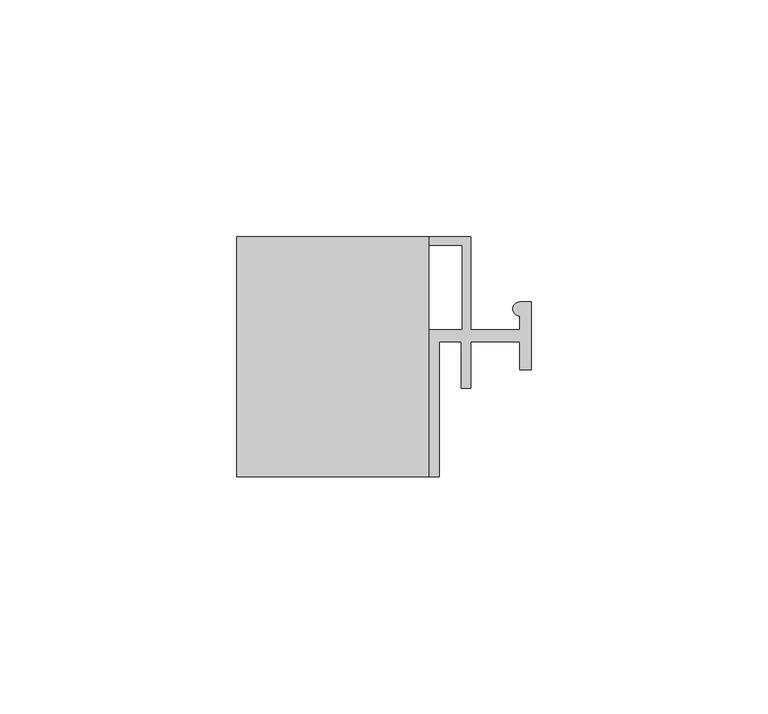
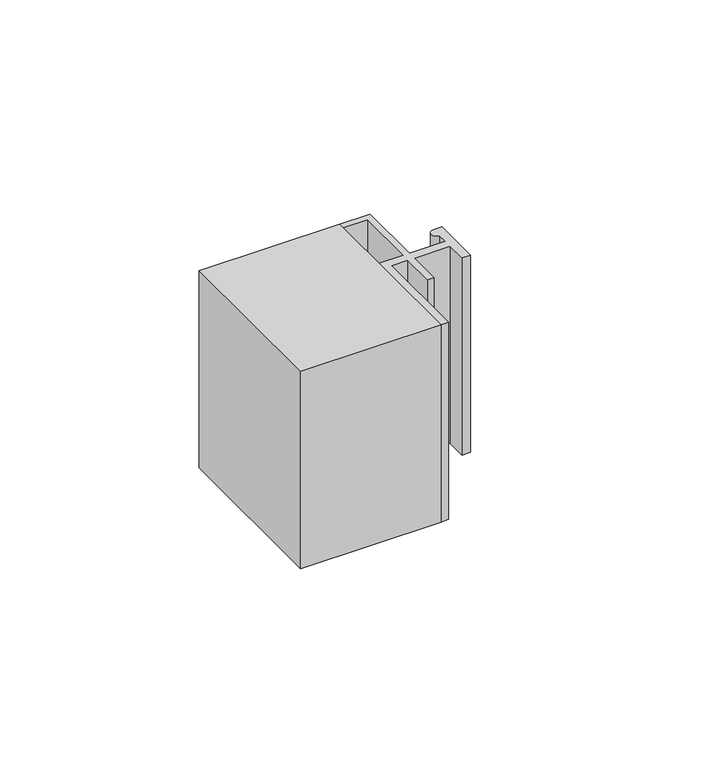
"""IFC4 building model written with IfcOpenShell, lengths in millimetres: proxy geometry, Generic Models 9:Generic Models 5:348123:Generic Models 5:348123 : Generic Models 9:Generic Models 5:348123:2 : Generic Models 9:Generic Models 5:348123:Generic Models 5:348123 : Generic Models 9:Generic Models 5:348123:301771."""

from ifc_helpers import new_model, si_unit, point, frame, frame_2d, origin, place, context, project, spatial, polyline, circle_curve, trimmed, segment, composite_curve, outline, extrude, source, transform, mapped, element, save


def generic_models_d8f6da72(model_context):
    return source(origin(), model_context, "Body", "SweptSolid", [
        extrude(outline(polyline([(32053.2090778, 39220.6364592), (32053.2090778, 39271.4364592), (32093.803738, 39271.4364592), (32093.803738, 39220.6364592), (32053.2090778, 39220.6364592)])), frame((0.0, 0.0, 267387.3875), z_axis=(0.0, 0.0, 1.0), x_axis=(1.0, 0.0, 0.0)), (0.0, 0.0, 1.0), 60.325),
        extrude(outline(composite_curve([segment(polyline([(32102.6814079, 39251.7083039), (32113.0386895, 39251.7083039), (32113.0386895, 39254.6675272)]), True, "CONTINUOUS"), segment(trimmed(circle_curve(frame_2d((32113.0386895, 39256.1471389)), 1.4796117), [point((32113.0386895, 39254.6675272))], [point((32113.0386895, 39257.6267505))], False, "CARTESIAN"), True, "CONTINUOUS"), segment(polyline([(32113.0386895, 39257.6267505), (32115.5047089, 39257.6267505), (32115.5047089, 39243.3238379), (32113.0386895, 39243.3238379), (32113.0386895, 39249.2422845), (32102.6814079, 39249.2422845), (32102.6814079, 39239.3782068), (32100.7085924, 39239.3782068), (32100.7085924, 39249.2422845), (32096.0724759, 39249.2422845), (32096.0724759, 39220.6364592), (32093.803738, 39220.6364592), (32093.803738, 39251.7083039), (32100.9058739, 39251.7083039), (32100.9058739, 39269.6609253), (32093.803738, 39269.6609253), (32093.803738, 39271.4364592), (32102.6814079, 39271.4364592), (32102.6814079, 39251.7083039)]), True, "CONTINUOUS")], self_intersect=False)), frame((0.0, 0.0, 267387.3875), z_axis=(0.0, 0.0, 1.0), x_axis=(1.0, 0.0, 0.0)), (0.0, 0.0, 1.0), 60.325),
    ])


if __name__ == "__main__":
    model = new_model("IFC4")
    model_context = context("Model", 3, world=origin())
    ifc_project = project(units=[si_unit("LENGTHUNIT", "METRE", prefix="MILLI")], contexts=[model_context])
    site = spatial("IfcSite", under=ifc_project)
    building = spatial("IfcBuilding", under=site)
    placement = place(None, origin())
    generic_models_shape = generic_models_d8f6da72(model_context)
    element("IfcBuildingElementProxy", 1, Name="Generic Models 9:Generic Models 5:348123:Generic Models 5:348123 : Generic Models 9:Generic Models 5:348123:2 : Generic Models 9:Generic Models 5:348123:Generic Models 5:348123 : Generic Models 9:Generic Models 5:348123:301771", ObjectType="Generic Models 9:Generic Models 5:348123:Generic Models 5:348123 : Generic Models 9:Generic Models 5:348123:2 : Generic Models 9:Generic Models 5:348123:Generic Models 5:348123 : Generic Models 9:Generic Models 5:348123:301771", at=placement, inside=building, context=model_context, shape_type="MappedRepresentation", body=[
        mapped(generic_models_shape, transform((0.0, 0.0, 0.0), x_axis=(1.0, 0.0, 0.0), y_axis=(0.0, 1.0, 0.0), z_axis=(0.0, 0.0, 1.0))),
    ])
    save(model, "model.ifc")

# Revit data of these elements
# Type "Generic Models 9:Generic Models 5:348123:Generic Models 5:348123 : Generic Models 9:Generic Models 5:348123:2 : Generic Models 9:Generic Models 5:348123:Generic Models 5:348123 : Generic Models 9:Generic Models 5:348123:301771"
#   NameOverride = "Generic Models 9:Generic Models 5:348123:Generic Models 5:348123 : Generic Models 9:Generic Models 5:348123:301771"
#   ObjectTypeOverride = "Generic Models 5:348123 : Generic Models 9:Generic Models 5:348123"
#   Reference = "Generic Models 5"
#   Tag = "301771"
# Element 1 (IfcBuildingElementProxy, "Generic Models 9:Generic Models 5:348123:Generic Models 5:348123 : Generic Models 9:Generic Models 5:348123:2 : Generic Models 9:Generic Models 5:348123:Generic Models 5:348123 : Generic Models 9:Generic Models 5:348123:301771")
#   Materials on its faces: "GA. STEEL CLIP AT EVERY SEAM IN POLYCARBONATE (WITH BLOCKING EXTENSIONS, IF NECS.)"
# Materials
#   "GA. STEEL CLIP AT EVERY SEAM IN POLYCARBONATE (WITH BLOCKING EXTENSIONS, IF NECS.)": class "Unassigned", colour RGB 120 120 120, transparency 0, Cost = 0
